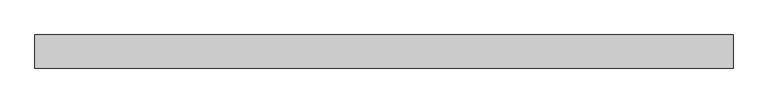
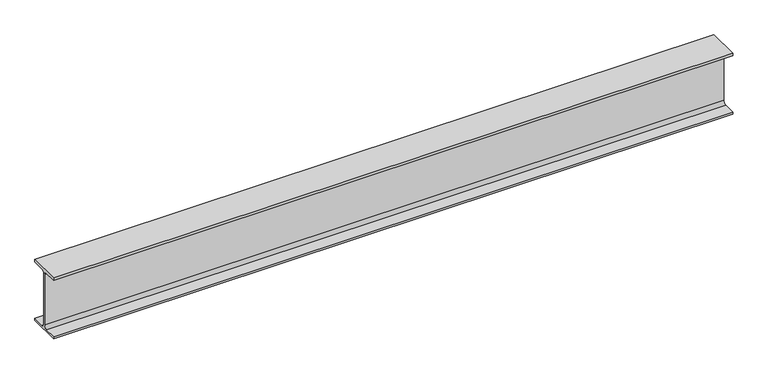
"""IFC4 building model written with IfcOpenShell, lengths in millimetres: beam geometry, 0912_Steel Framing_H-KSD3502 : H_SB_ASB_H-250x125x6x9."""

from ifc_helpers import new_model, si_unit, point, frame, frame_2d, origin, place, context, project, spatial, polyline, circle_curve, trimmed, segment, composite_curve, outline, extrude, source, transform, mapped, element, save


def beam_dbfcdd3c(model_context):
    return source(origin(), model_context, "Body", "SweptSolid", [
        extrude(outline(composite_curve([segment(polyline([(62.5, -116.0), (62.5, -125.0), (-62.5, -125.0), (-62.5, -116.0), (-15.0, -116.0)]), True, "CONTINUOUS"), segment(trimmed(circle_curve(frame_2d((-15.0, -104.0)), 12.0), [point((-15.0, -116.0))], [point((-3.0, -104.0))], True, "CARTESIAN"), True, "CONTINUOUS"), segment(polyline([(-3.0, -104.0), (-3.0, 104.0)]), True, "CONTINUOUS"), segment(trimmed(circle_curve(frame_2d((-15.0, 104.0)), 12.0), [point((-3.0, 104.0))], [point((-15.0, 116.0))], True, "CARTESIAN"), True, "CONTINUOUS"), segment(polyline([(-15.0, 116.0), (-62.5, 116.0), (-62.5, 125.0), (62.5, 125.0), (62.5, 116.0), (15.0, 116.0)]), True, "CONTINUOUS"), segment(trimmed(circle_curve(frame_2d((15.0, 104.0)), 12.0), [point((15.0, 116.0))], [point((3.0, 104.0))], True, "CARTESIAN"), True, "CONTINUOUS"), segment(polyline([(3.0, 104.0), (3.0, -104.0)]), True, "CONTINUOUS"), segment(trimmed(circle_curve(frame_2d((15.0, -104.0)), 12.0), [point((3.0, -104.0))], [point((15.0, -116.0))], True, "CARTESIAN"), True, "CONTINUOUS"), segment(polyline([(15.0, -116.0), (62.5, -116.0)]), True, "CONTINUOUS")], self_intersect=False)), frame((-1249.3, 0.0, 0.0), z_axis=(1.0, 0.0, 0.0), x_axis=(0.0, 1.0, 0.0)), (0.0, 0.0, 1.0), 2636.6),
    ])


if __name__ == "__main__":
    model = new_model("IFC4")
    model_context = context("Model", 3, world=origin())
    ifc_project = project(units=[si_unit("LENGTHUNIT", "METRE", prefix="MILLI")], contexts=[model_context])
    site = spatial("IfcSite", under=ifc_project)
    building = spatial("IfcBuilding", under=site)
    placement = place(None, origin())
    beam_shape = beam_dbfcdd3c(model_context)
    element("IfcBeam", 1, ObjectType="0912_Steel Framing_H-KSD3502 : H_SB_ASB_H-250x125x6x9", at=placement, inside=building, context=model_context, shape_type="MappedRepresentation", body=[
        mapped(beam_shape, transform((0.0, 0.0, 0.0), x_axis=(1.0, 0.0, 0.0), y_axis=(0.0, 1.0, 0.0), z_axis=(0.0, 0.0, 1.0))),
    ])
    save(model, "model.ifc")

# Revit data of these elements
# Type "0912_Steel Framing_H-KSD3502 : H_SB_ASB_H-250x125x6x9"
#   H_WM Code_1 = "S01AA003-00001 | Main Steel Structure Fabrication Work | Shelter/Building | Light Steel - Standard (30KG/M>Weight) | Material: (   )"
#   H_WM Code_2 = "S03AA029-00001 | Main Steel Structure Erection Work | Shelter/Building | Light Steel (30KG/M>Weight) | Material: (   )"
#   H_WM Code_3 = "S01AA010-00001 | Main Steel Structure Fabrication Work | Shelter/Building | Steel Painting/Coating | for Non-Fireproofed Steel Surface, Surface Preparation, Primer, Second & Final Coat | Material: (   )"
#   H_Q'ty Cal Type Tag = "SB-Q2"
#   Width = 12.5 cm
#   Web Thickness = 0.6 cm
#   Web Fillet = 1.2 cm
#   Warping Constant = 42539.8 cm⁶
#   W = 0
#   Torsional Moment of Inertia = 7.8102 cm⁴
#   Section Area = 37.66 cm²
#   Plastic Modulus weak axis = 73.1 cm³
#   Plastic Modulus strong axis = 366.0 cm³
#   Perimeter = 0.97 m²/m
#   Nominal Weight = 29.60 kgf/m
#   Moment of Inertia weak axis = 294.00 cm⁴
#   Moment of Inertia strong axis = 4050.00 cm⁴
#   Height = 25.0 cm
#   Flange Thickness = 0.9 cm
#   Elastic Modulus weak axis = 47.0 cm³
#   Elastic Modulus strong axis = 324.0 cm³
#   Centroid Vertical = 12.5 cm
#   Centroid Horizontal = 6.25 cm
#   Ix = 40500000
#   Length [instance default] = 1.5240 m
#   Zx = 366000
#   b = 0.1250 m
#   h = 0.2500 m
#   r = 0.0120 m
#   s = 0.0060 m
#   t = 0.0090 m
#   A = 0.003766 m²
#   Structural Material [instance default] = Steel, 45-345
#   Assembly Code = ""
# Element 1 (IfcBeam, "0912_Steel Framing_H-KSD3502 : H_SB_ASB_H-250x125x6x9")
#   Structural Material = none
# Materials
#   "Steel, 45-345": class "Metal", colour RGB 189 187 185, transparency 0, Description = "Steel 345 MPa", Cost = 0
